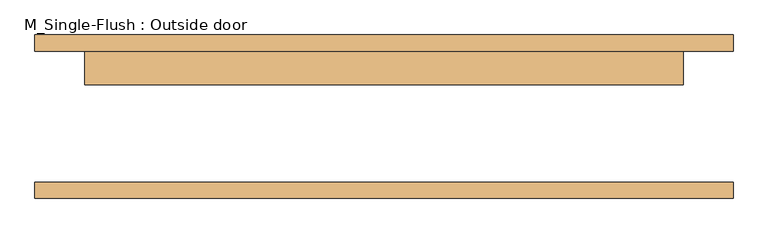
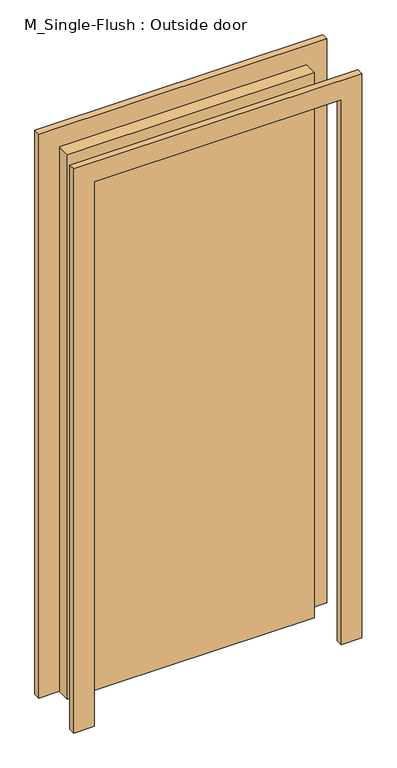
"""IFC4 building model written with IfcOpenShell, lengths in millimetres: door geometry, M_Single-Flush : Outside door."""

from ifc_helpers import new_model, si_unit, frame, origin, origin_with_axes, place, context, project, spatial, polyline, outline, extrude, source, transform, mapped, element, save


def m_single_flush_outside_door_6a9e8738(model_context):
    return source(origin(), model_context, "Body", "SweptSolid", [
        extrude(outline(polyline([(2210.0, -533.5), (0.0, -533.5), (0.0, -457.5), (2134.0, -457.5), (2134.0, 457.5), (0.0, 457.5), (0.0, 533.5), (2210.0, 533.5), (2210.0, -533.5)])), frame((0.0, 100.0, 0.0), z_axis=(0.0, 1.0, 0.0), x_axis=(0.0, 0.0, 1.0)), (0.0, 0.0, 1.0), 25.0),
        extrude(outline(polyline([(2210.0, 533.5), (2210.0, -533.5), (0.0, -533.5), (0.0, -457.5), (2134.0, -457.5), (2134.0, 457.5), (0.0, 457.5), (0.0, 533.5), (2210.0, 533.5)])), frame((0.0, -125.0, 0.0), z_axis=(0.0, 1.0, 0.0), x_axis=(0.0, 0.0, 1.0)), (0.0, 0.0, 1.0), 25.0),
        extrude(outline(polyline([(457.5, 49.0), (-457.5, 49.0), (-457.5, 100.0), (457.5, 100.0), (457.5, 49.0)])), origin_with_axes(), (0.0, 0.0, 1.0), 2134.0),
    ])


if __name__ == "__main__":
    model = new_model("IFC4")
    model_context = context("Model", 3, world=origin())
    ifc_project = project(units=[si_unit("LENGTHUNIT", "METRE", prefix="MILLI")], contexts=[model_context])
    site = spatial("IfcSite", under=ifc_project)
    building = spatial("IfcBuilding", under=site)
    placement = place(None, origin())
    m_single_flush_outside_door_shape = m_single_flush_outside_door_6a9e8738(model_context)
    element("IfcDoor", 1, ObjectType="M_Single-Flush : Outside door", at=placement, inside=building, context=model_context, shape_type="MappedRepresentation", body=[
        mapped(m_single_flush_outside_door_shape, transform((0.0, 0.0, 0.0), x_axis=(1.0, 0.0, 0.0), y_axis=(0.0, 1.0, 0.0), z_axis=(0.0, 0.0, 1.0))),
    ])
    save(model, "model.ifc")

# Revit data of these elements
# Project information
#   Organization Name = "// ORGANIZATION/NAME //"
#   Organization Description = "// ORGANIZATION/DESCRIPTION //"
#   Building Name = "// BUILDING/NAME //"
#   Author = "// AUTHOR //"
#   Project Issue Date = "// ISSUE DATE //"
#   Project Status = "// PROJECT/STATUS //"
#   Client Name = "// CLIENT/NAME //"
#   Project Address = "Enter address here"
#   Project Name = "// PROJECT/NAME //"
#   Project Number = "// PROJECT/NUMBER //"
# Type "M_Single-Flush : Outside door"
#   Keynote = "--KEYNOTE--"
#   Model = "--MODEL--"
#   Manufacturer = "--TYPE_COMMENTS_"
#   URL = "--URL--"
#   Description = "--DESCRIPTION--"
#   Assembly Code = "--ASSEMBLY_CODE--"
#   Type Mark = "20"
#   Operation = "--OPERATION--"
#   Fire Rating = "--FIRE_CODE--"
#   Construction Type Id = "MDOOR"
#   Analytic Construction = "Metal"
#   Thickness = 51 mm
#   Thermal Resistance (R) = 0.270117 (m²·K)/W
#   Heat Transfer Coefficient (U) = 3.7021 W/(m²·K)
#   Height = 2134 mm
#   Trim Projection Ext = 25 mm
#   Trim Projection Int = 25 mm
#   Trim Width = 76 mm
#   Width = 915 mm
#   Define Thermal Properties by = 1
#   Define Thermal Properties by = 1
#   Door Material = Door - Panel
#   Frame Material = Door - Frame
#   Visual Light Transmittance = 0
#   Solar Heat Gain Coefficient = 0
#   Function = (empty or 0)
#   Wall Closure = (empty or 0)
# Element 1 (IfcDoor, "M_Single-Flush : Outside door")
#   Materials on its faces: "Door - Frame", "Door - Panel"
# Materials
#   "Door - Panel": class "Wood", colour RGB 210 159 95, transparency 0, Cost = 0
#   "Door - Frame": class "Miscellaneous", colour RGB 118 70 51, transparency 0, Cost = 0
